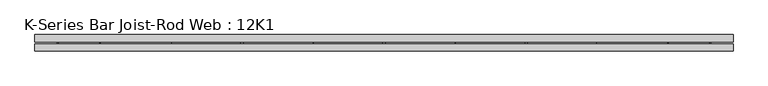
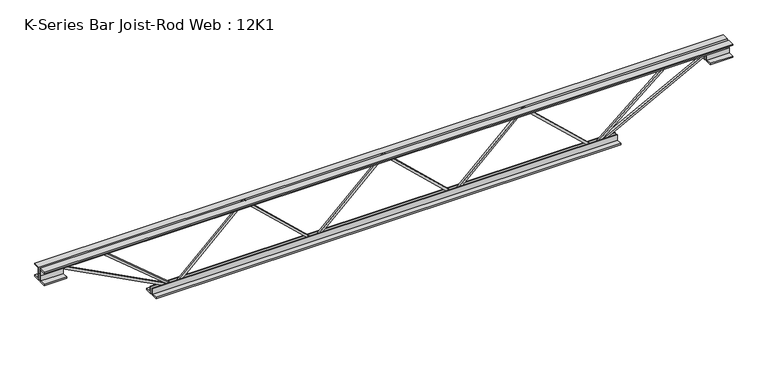
"""IFC4 building model written with IfcOpenShell, lengths in millimetres: beam geometry, K-Series Bar Joist-Rod Web : 12K1."""

import ifcopenshell
import ifcopenshell.guid

model = None  # the IFC model being written
_history = None  # IfcOwnerHistory: only IFC2X3 demands one
_inside = {}  # id of a spatial element -> (the spatial element, [elements in it])
_under = {}  # id of a project, library or spatial element -> (it, [spatial elements below it])
_declared = {}  # id of a project -> (the project, [libraries it declares])
_typed = {}  # id of a type object -> (the type object, [elements of that type])
_made_of = {}  # id of a material, layer set ... -> (it, [elements and type objects made of it])


def new_model(schema):
    """Start an empty IFC model of exactly this schema.

    Asked for "IFC4X3", IfcOpenShell would pick the latest addendum, in which some entities
    have other attributes; the version numbers below select the first issue.
    IFC2X3 requires an IfcOwnerHistory on every rooted entity: one is made here for all.
    """
    global model, _history
    if schema == "IFC4X3":
        model = ifcopenshell.file(schema_version=(4, 3, 0, 0))
    else:
        model = ifcopenshell.file(schema=schema)
    _inside.clear()
    _under.clear()
    _declared.clear()
    _typed.clear()
    _made_of.clear()
    _history = None
    if model.schema == "IFC2X3":
        org = make("IfcOrganization", Name="unknown")
        user = make(
            "IfcPersonAndOrganization",
            ThePerson=make("IfcPerson", FamilyName="unknown"),
            TheOrganization=org,
        )
        app = make(
            "IfcApplication",
            ApplicationDeveloper=org,
            Version="unknown",
            ApplicationFullName="unknown",
            ApplicationIdentifier="unknown",
        )
        _history = make(
            "IfcOwnerHistory",
            OwningUser=user,
            OwningApplication=app,
            ChangeAction="ADDED",
            CreationDate=0,
        )
    return model


def make(cls, **values):
    """One entity of the class cls with the attributes given. An attribute that is None is left unset."""
    return model.create_entity(
        cls, **{name: value for name, value in values.items() if value is not None}
    )


def rooted(cls, **values):
    """An entity with a GlobalId (a new one), such as an element, a storey or a relation."""
    return make(cls, GlobalId=ifcopenshell.guid.new(), OwnerHistory=_history, **values)


def si_unit(unit_type, name, prefix=None):
    """IfcSIUnit, for example si_unit("LENGTHUNIT", "METRE", prefix="MILLI")."""
    return make("IfcSIUnit", UnitType=unit_type, Prefix=prefix, Name=name)


def assignment(units):
    """IfcUnitAssignment: the units of a project."""
    return None if units is None else make("IfcUnitAssignment", Units=units)


def point(xyz):
    """IfcCartesianPoint."""
    return None if xyz is None else make("IfcCartesianPoint", Coordinates=xyz)


def direction(xyz):
    """IfcDirection."""
    return None if xyz is None else make("IfcDirection", DirectionRatios=xyz)


def frame(location, z_axis=None, x_axis=None):
    """IfcAxis2Placement3D, a coordinate frame: its origin and axes. An axis left out is left unset."""
    return make(
        "IfcAxis2Placement3D",
        Location=point(location),
        Axis=direction(z_axis),
        RefDirection=direction(x_axis),
    )


def origin():
    """The frame at (0, 0, 0) with its axes left unset."""
    return frame((0.0, 0.0, 0.0))


def place(relative_to, where):
    """IfcLocalPlacement: puts the frame where relative to a parent placement (None: the world)."""
    return make(
        "IfcLocalPlacement", PlacementRelTo=relative_to, RelativePlacement=where
    )


def context(
    kind, dimensions, precision=None, world=None, true_north=None, identifier=None
):
    """IfcGeometricRepresentationContext, for example the 3D "Model" context."""
    return make(
        "IfcGeometricRepresentationContext",
        ContextIdentifier=identifier,
        ContextType=kind,
        CoordinateSpaceDimension=dimensions,
        Precision=precision,
        WorldCoordinateSystem=world,
        TrueNorth=true_north,
    )


def project(units=None, contexts=None):
    """IfcProject with its units and contexts."""
    return rooted(
        "IfcProject",
        Name="project",
        RepresentationContexts=contexts,
        UnitsInContext=assignment(units),
    )


def spatial(cls, under=None, at=None, **own):
    """A site, building, storey or space (cls), placed at a placement, below another one or the project."""
    s = rooted(cls, ObjectPlacement=at, **own)
    if under is not None:
        _under.setdefault(under.id(), (under, []))[1].append(s)
    return s


def polyline(points):
    """IfcPolyline through the points."""
    return make("IfcPolyline", Points=[point(p) for p in points])


def outline(outer, holes=None, kind="AREA"):
    """IfcArbitraryClosedProfileDef: a profile drawn as a closed curve; with holes, ...WithVoids."""
    if holes is None:
        return make("IfcArbitraryClosedProfileDef", ProfileType=kind, OuterCurve=outer)
    return make(
        "IfcArbitraryProfileDefWithVoids",
        ProfileType=kind,
        OuterCurve=outer,
        InnerCurves=holes,
    )


def extrude(swept, where, along, depth):
    """IfcExtrudedAreaSolid: the profile swept, set in the frame where, extruded along a direction by depth."""
    return make(
        "IfcExtrudedAreaSolid",
        SweptArea=swept,
        Position=where,
        ExtrudedDirection=direction(along),
        Depth=depth,
    )


def shape(context_of_items, identifier, shape_type, items):
    """IfcShapeRepresentation: the items that make up one representation, for example the "Body"."""
    return make(
        "IfcShapeRepresentation",
        ContextOfItems=context_of_items,
        RepresentationIdentifier=identifier,
        RepresentationType=shape_type,
        Items=items,
    )


def source(mapping_origin, context_of_items, identifier, shape_type, items):
    """IfcRepresentationMap: a shape defined once, which mapped items show again and again."""
    return make(
        "IfcRepresentationMap",
        MappingOrigin=mapping_origin,
        MappedRepresentation=shape(context_of_items, identifier, shape_type, items),
    )


def transform(
    local_origin,
    x_axis=None,
    y_axis=None,
    z_axis=None,
    scale=None,
    scale2=None,
    scale3=None,
    uniform=True,
):
    """IfcCartesianTransformationOperator3D, or its non-uniform kind. x_axis, y_axis, z_axis: its Axis1, 2, 3."""
    if uniform:
        return make(
            "IfcCartesianTransformationOperator3D",
            Axis1=direction(x_axis),
            Axis2=direction(y_axis),
            LocalOrigin=point(local_origin),
            Scale=scale,
            Axis3=direction(z_axis),
        )
    return make(
        "IfcCartesianTransformationOperator3DnonUniform",
        Axis1=direction(x_axis),
        Axis2=direction(y_axis),
        LocalOrigin=point(local_origin),
        Scale=scale,
        Axis3=direction(z_axis),
        Scale2=scale2,
        Scale3=scale3,
    )


def mapped(mapping_source, mapping_target):
    """IfcMappedItem: shows the shape of a source again, moved by a transform."""
    return make(
        "IfcMappedItem", MappingSource=mapping_source, MappingTarget=mapping_target
    )


def made_of(thing, what):
    """Note that an element or type object is made of a material, layer set ...; save() writes the relation."""
    if what is not None:
        _made_of.setdefault(what.id(), (what, []))[1].append(thing)
    return thing


def element(
    cls,
    number,
    at=None,
    inside=None,
    cuts=None,
    type_object=None,
    material=None,
    context=None,
    identifier="Body",
    shape_type=None,
    held_by="IfcProductDefinitionShape",
    body=None,
    shapes=None,
    **own,
):
    """One element of the class cls, such as IfcWall. Its Tag is "e" and its number.

    at: its placement. inside: the storey or other place that contains it. cuts: it is an
    opening in that element (IfcRelVoidsElement). A single representation is given by context,
    identifier, shape_type and body (its items); several are given by shapes. held_by: the class
    of the entity that holds the representations. save() writes the other relations.
    """
    e = rooted(cls, Tag="e%d" % number, ObjectPlacement=at, **own)
    if body is not None:
        shapes = [shape(context, identifier, shape_type, body)]
    if shapes is not None:
        e.Representation = make(held_by, Representations=shapes)
    if inside is not None:
        _inside.setdefault(inside.id(), (inside, []))[1].append(e)
    if cuts is not None:
        rooted(
            "IfcRelVoidsElement", RelatingBuildingElement=cuts, RelatedOpeningElement=e
        )
    if type_object is not None:
        _typed.setdefault(type_object.id(), (type_object, []))[1].append(e)
    return made_of(e, material)


def aggregate(whole, parts):
    """IfcRelAggregates: a whole, such as a stair, and the parts it consists of."""
    return rooted("IfcRelAggregates", RelatingObject=whole, RelatedObjects=parts)


def save(model, path):
    """Write the relations noted so far, then the file.

    IfcRelAggregates (storeys below a building ...), IfcRelContainedInSpatialStructure (elements
    in a storey), IfcRelDefinesByType, IfcRelAssociatesMaterial and IfcRelDeclares: one each for
    every whole, place, type object, material and project.
    """
    for whole, parts in _under.values():
        aggregate(whole, parts)
    for where, things in _inside.values():
        rooted(
            "IfcRelContainedInSpatialStructure",
            RelatedElements=things,
            RelatingStructure=where,
        )
    for kind, things in _typed.values():
        rooted("IfcRelDefinesByType", RelatedObjects=things, RelatingType=kind)
    for what, things in _made_of.values():
        rooted("IfcRelAssociatesMaterial", RelatedObjects=things, RelatingMaterial=what)
    for by, libraries in _declared.values():
        rooted("IfcRelDeclares", RelatingContext=by, RelatedDefinitions=libraries)
    model.write(path)


def k_series_bar_joist_rod_web_12k1_546f384c(model_context):
    return source(origin(), model_context, "Body", "SweptSolid", [
        extrude(outline(polyline([(-141.2875, -317.5), (-150.8125, -317.5), (-150.8125, -312.439813), (141.2875, -1.289813), (141.2875, 1.289813), (-150.8125, 312.439813), (-150.8125, 317.5), (-141.2875, 317.5), (-141.2875, 316.210187), (150.8125, 5.060187), (150.8125, -5.060187), (-141.2875, -316.210187), (-141.2875, -317.5)])), frame((0.0, -4.7625, 0.0), z_axis=(0.0, 1.0, 0.0), x_axis=(0.0, 0.0, 1.0)), (0.0, 0.0, 1.0), 9.525),
        extrude(outline(polyline([(-141.2875, 317.5), (-150.8125, 317.5), (-150.8125, 322.560187), (141.2875, 633.710187), (141.2875, 636.289813), (-150.8125, 947.439813), (-150.8125, 952.5), (-141.2875, 952.5), (-141.2875, 951.210187), (150.8125, 640.060187), (150.8125, 629.939813), (-141.2875, 318.789813), (-141.2875, 317.5)])), frame((0.0, -4.7625, 0.0), z_axis=(0.0, 1.0, 0.0), x_axis=(0.0, 0.0, 1.0)), (0.0, 0.0, 1.0), 9.525),
        extrude(outline(polyline([(-141.2875, -952.5), (-150.8125, -952.5), (-150.8125, -947.439813), (141.2875, -636.289813), (141.2875, -633.710187), (-150.8125, -322.560187), (-150.8125, -317.5), (-141.2875, -317.5), (-141.2875, -318.789813), (150.8125, -629.939813), (150.8125, -640.060187), (-141.2875, -951.210187), (-141.2875, -952.5)])), frame((0.0, -4.7625, 0.0), z_axis=(0.0, 1.0, 0.0), x_axis=(0.0, 0.0, 1.0)), (0.0, 0.0, 1.0), 9.525),
        extrude(outline(polyline([(4.7625, 152.4), (36.5125, 152.4), (36.5125, 146.05), (11.1125, 146.05), (11.1125, 120.65), (4.7625, 120.65), (4.7625, 152.4)])), frame((-1562.1, 0.0, 0.0), z_axis=(1.0, 0.0, 0.0), x_axis=(0.0, 1.0, 0.0)), (0.0, 0.0, 1.0), 3124.2),
        extrude(outline(polyline([(-4.7625, 152.4), (-4.7625, 120.65), (-11.1125, 120.65), (-11.1125, 146.05), (-36.5125, 146.05), (-36.5125, 152.4), (-4.7625, 152.4)])), frame((-1562.1, 0.0, 0.0), z_axis=(1.0, 0.0, 0.0), x_axis=(0.0, 1.0, 0.0)), (0.0, 0.0, 1.0), 3124.2),
        extrude(outline(polyline([(-4.7625, 88.9), (-36.5125, 88.9), (-36.5125, 95.25), (-11.1125, 95.25), (-11.1125, 120.65), (-4.7625, 120.65), (-4.7625, 88.9)])), frame((-1562.1, 0.0, 0.0), z_axis=(1.0, 0.0, 0.0), x_axis=(0.0, 1.0, 0.0)), (0.0, 0.0, 1.0), 101.6),
        extrude(outline(polyline([(36.5125, 88.9), (4.7625, 88.9), (4.7625, 120.65), (11.1125, 120.65), (11.1125, 95.25), (36.5125, 95.25), (36.5125, 88.9)])), frame((-1562.1, 0.0, 0.0), z_axis=(1.0, 0.0, 0.0), x_axis=(0.0, 1.0, 0.0)), (0.0, 0.0, 1.0), 101.6),
        extrude(outline(polyline([(4.7625, 88.9), (4.7625, 120.65), (11.1125, 120.65), (11.1125, 95.25), (36.5125, 95.25), (36.5125, 88.9), (4.7625, 88.9)])), frame((1460.5, 0.0, 0.0), z_axis=(1.0, 0.0, 0.0), x_axis=(0.0, 1.0, 0.0)), (0.0, 0.0, 1.0), 101.6),
        extrude(outline(polyline([(-4.7625, 88.9), (-36.5125, 88.9), (-36.5125, 95.25), (-11.1125, 95.25), (-11.1125, 120.65), (-4.7625, 120.65), (-4.7625, 88.9)])), frame((1460.5, 0.0, 0.0), z_axis=(1.0, 0.0, 0.0), x_axis=(0.0, 1.0, 0.0)), (0.0, 0.0, 1.0), 101.6),
        extrude(outline(polyline([(4.7625, -152.4), (4.7625, -120.65), (11.1125, -120.65), (11.1125, -146.05), (36.5125, -146.05), (36.5125, -152.4), (4.7625, -152.4)])), frame((-1054.1, 0.0, 0.0), z_axis=(1.0, 0.0, 0.0), x_axis=(0.0, 1.0, 0.0)), (0.0, 0.0, 1.0), 2108.2),
        extrude(outline(polyline([(-4.7625, -152.4), (-36.5125, -152.4), (-36.5125, -146.05), (-11.1125, -146.05), (-11.1125, -120.65), (-4.7625, -120.65), (-4.7625, -152.4)])), frame((-1054.1, 0.0, 0.0), z_axis=(1.0, 0.0, 0.0), x_axis=(0.0, 1.0, 0.0)), (0.0, 0.0, 1.0), 2108.2),
        extrude(outline(polyline([(0.0, -9.525), (0.0, 0.0), (573.7533355, 0.0), (573.7533355, -9.525), (0.0, -9.525)])), frame((-1462.7137714, 4.7625, 116.4332925), z_axis=(0.46483389898951416, 0.0, 0.8853979028381568), x_axis=(0.8853979028381568, 0.0, -0.46483389898951416)), (0.0, 0.0, 1.0), 9.525),
        extrude(outline(polyline([(0.0, -9.525), (0.0, 0.0), (414.650624, 0.0), (414.650624, -9.525), (0.0, -9.525)])), frame((-1273.0632023, 4.7625, 117.0033306), z_axis=(0.6431920864228818, 0.0, 0.7657048647899398), x_axis=(0.7657048647899398, 0.0, -0.6431920864228818)), (0.0, 0.0, 1.0), 9.525),
        extrude(outline(polyline([(0.0, -9.525), (0.0, 0.0), (573.7533355, 0.0), (573.7533355, -9.525), (0.0, -9.525)])), frame((1462.7137714, -4.7625, 116.4332925), z_axis=(-0.4648338989894944, 0.0, 0.8853979028381672), x_axis=(-0.8853979028381672, 0.0, -0.4648338989894944)), (0.0, 0.0, 1.0), 9.525),
        extrude(outline(polyline([(0.0, -9.525), (0.0, 0.0), (414.650624, 0.0), (414.650624, -9.525), (0.0, -9.525)])), frame((1273.0632023, -4.7625, 117.0033306), z_axis=(-0.6431920864228763, 0.0, 0.7657048647899446), x_axis=(-0.7657048647899446, 0.0, -0.6431920864228763)), (0.0, 0.0, 1.0), 9.525),
    ])


if __name__ == "__main__":
    model = new_model("IFC4")
    model_context = context("Model", 3, world=origin())
    ifc_project = project(units=[si_unit("LENGTHUNIT", "METRE", prefix="MILLI")], contexts=[model_context])
    site = spatial("IfcSite", under=ifc_project)
    building = spatial("IfcBuilding", under=site)
    placement = place(None, origin())
    k_series_bar_joist_rod_web_12k1_shape = k_series_bar_joist_rod_web_12k1_546f384c(model_context)
    element("IfcBeam", 1, ObjectType="K-Series Bar Joist-Rod Web : 12K1", at=placement, inside=building, context=model_context, shape_type="MappedRepresentation", body=[
        mapped(k_series_bar_joist_rod_web_12k1_shape, transform((0.0, 0.0, 0.0), x_axis=(1.0, 0.0, 0.0), y_axis=(0.0, 1.0, 0.0), z_axis=(0.0, 0.0, 1.0))),
    ])
    save(model, "model.ifc")

# Revit data of these elements
# Type "K-Series Bar Joist-Rod Web : 12K1"
#   Assembly Code = "B1010350"
#   Wt = 5
#   Web Thickness = 0' - 0 3/8"
#   Start Offset [instance default] = 0' - 0"
#   Start Extension [instance default] = 0' - 0"
#   Seat Length = 0' - 4"
#   Seat Depth = 0' - 2 1/2"
#   PanelArrayLength [instance default] = 20' - 0"
#   Panel [instance default] = 2' - 0"
#   End Offset [instance default] = 0' - 0"
#   End Extension [instance default] = 0' - 0"
#   End Panel = 2' - 0"
#   Cord Leg = 0' - 1 1/4"
#   Chord Thickness = 0' - 0 1/4"
#   Length [instance default] = 24' - 0"
#   Depth = 1' - 0"
#   PanelArrayNum [instance default] = 10
#   Structural Material = none
# Element 1 (IfcBeam, "K-Series Bar Joist-Rod Web : 12K1")
#   PanelArrayLength = 6' - 3"
#   Panel = 2' - 1"
#   PanelArrayNum = 3
